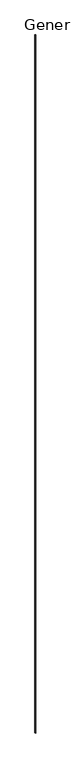
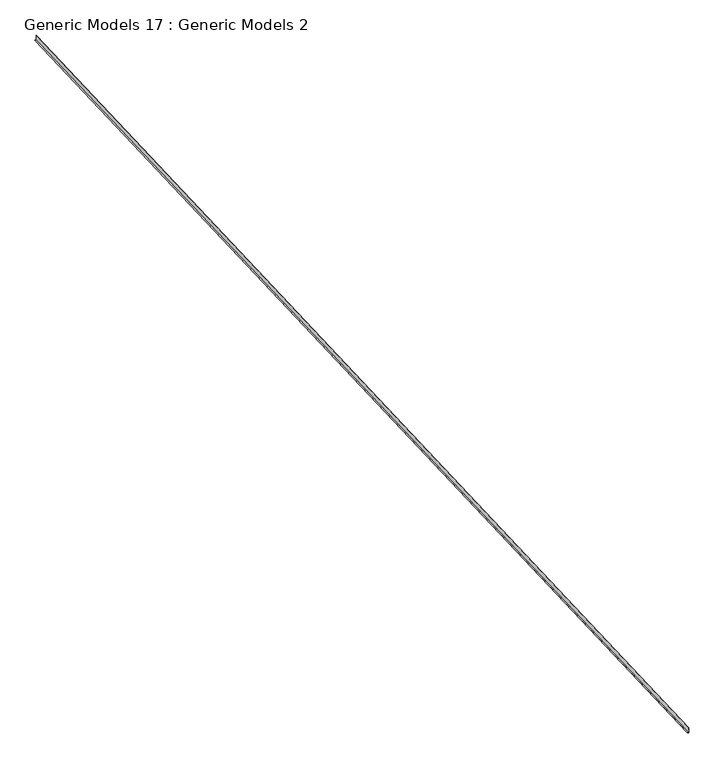
"""IFC4 building model written with IfcOpenShell, lengths in millimetres: proxy geometry, Generic Models 17 : Generic Models 2."""

from ifc_helpers import new_model, si_unit, frame, origin, place, context, project, spatial, polyline, outline, extrude, source, transform, mapped, element, save


def generic_models_17_generic_models_2_d9b7711a(model_context):
    return source(origin(), model_context, "Body", "SweptSolid", [
        extrude(outline(polyline([(-120.6499999, 0.0), (29.9148182, 0.0), (29.9148182, -1.5875), (-119.0625, -1.5875), (-119.0625, -38.1), (-120.6499999, -38.1), (-120.6499999, 0.0)])), frame((667550.8330405, -569981.0593115, 8810.6182088), z_axis=(0.0, 0.9991330730923521, 0.041630544712176844), x_axis=(0.0, -0.041630544712176844, 0.9991330730923521)), (0.0, 0.0, 1.0), 33406.7702703),
    ])


if __name__ == "__main__":
    model = new_model("IFC4")
    model_context = context("Model", 3, world=origin())
    ifc_project = project(units=[si_unit("LENGTHUNIT", "METRE", prefix="MILLI")], contexts=[model_context])
    site = spatial("IfcSite", under=ifc_project)
    building = spatial("IfcBuilding", under=site)
    placement = place(None, origin())
    generic_models_17_generic_models_2_shape = generic_models_17_generic_models_2_d9b7711a(model_context)
    element("IfcBuildingElementProxy", 1, Name="Generic Models 17 : Generic Models 2", ObjectType="Generic Models 17 : Generic Models 2", at=placement, inside=building, context=model_context, shape_type="MappedRepresentation", body=[
        mapped(generic_models_17_generic_models_2_shape, transform((0.0, 0.0, 0.0), x_axis=(1.0, 0.0, 0.0), y_axis=(0.0, 1.0, 0.0), z_axis=(0.0, 0.0, 1.0))),
    ])
    save(model, "model.ifc")

# Revit data of these elements
# Element 1 (IfcBuildingElementProxy, "Generic Models 17 : Generic Models 2")
#   Materials on its faces: "RAKE SUPPORT ANGLE - SEE STRUCT. DWGs"
# Materials
#   "RAKE SUPPORT ANGLE - SEE STRUCT. DWGs": class "Unassigned", colour RGB 210 209 208, transparency 0, Cost = 0
